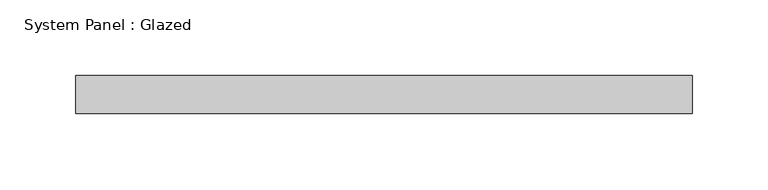
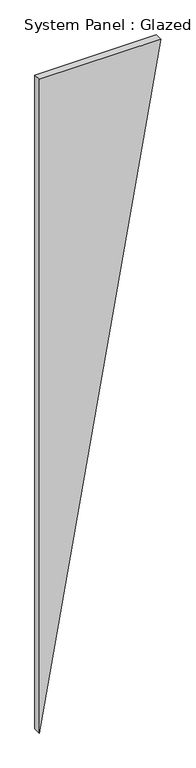
"""IFC4 building model written with IfcOpenShell, lengths in millimetres: plate geometry, System Panel : Glazed."""

from ifc_helpers import new_model, si_unit, frame, origin, place, context, project, spatial, polyline, outline, extrude, source, transform, mapped, element, save


def system_panel_glazed_96c5221b(model_context):
    return source(origin(), model_context, "Body", "SweptSolid", [
        extrude(outline(polyline([(0.0, -204.2314386), (2325.3567738, 204.2314386), (2325.3567738, -204.2314386), (0.0, -204.2314386)])), frame((0.0, -44.45, 0.0), z_axis=(0.0, 1.0, 0.0), x_axis=(0.0, 0.0, 1.0)), (0.0, 0.0, 1.0), 25.4),
    ])


if __name__ == "__main__":
    model = new_model("IFC4")
    model_context = context("Model", 3, world=origin())
    ifc_project = project(units=[si_unit("LENGTHUNIT", "METRE", prefix="MILLI")], contexts=[model_context])
    site = spatial("IfcSite", under=ifc_project)
    building = spatial("IfcBuilding", under=site)
    placement = place(None, origin())
    system_panel_glazed_shape = system_panel_glazed_96c5221b(model_context)
    element("IfcPlate", 1, ObjectType="System Panel : Glazed", at=placement, inside=building, context=model_context, shape_type="MappedRepresentation", body=[
        mapped(system_panel_glazed_shape, transform((0.0, 0.0, 0.0), x_axis=(1.0, 0.0, 0.0), y_axis=(0.0, 1.0, 0.0), z_axis=(0.0, 0.0, 1.0))),
    ])
    save(model, "model.ifc")

# Revit data of these elements
# Type "System Panel : Glazed"
#   Construction Type Id = "GSP4R"
#   Analytic Construction = "1/8 in Pilkington single glazing"
#   Visual Light Transmittance = 0.9
#   Solar Heat Gain Coefficient = 0.86
#   Heat Transfer Coefficient (U) = 1.18115 BTU/(h·ft²·°F)
#   Define Thermal Properties by = 1
# Element 1 (IfcPlate, "System Panel : Glazed")
#   Materials on its faces: "Glass"
# Materials
#   "Glass": class "Glass", colour RGB 0 128 192, transparency 0.75, Description = "Soda Lime Glass", Cost = 0
